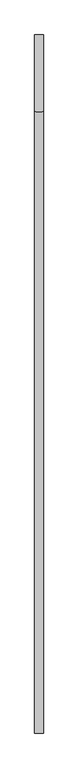
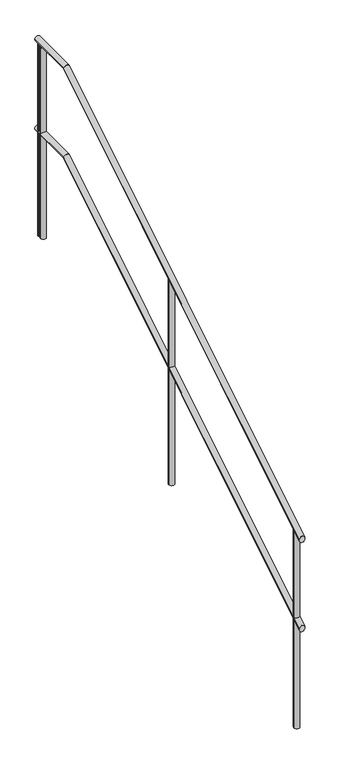
"""IFC4 building model written with IfcOpenShell, lengths in millimetres: railing geometry."""

from ifc_helpers import new_model, si_unit, point, frame, frame_2d, origin, place, context, project, spatial, circle_curve, ellipse_curve, trimmed, segment, composite_curve, outline, extrude, source, transform, mapped, element, save
from ifc_brep_helpers import plane_surface, cylinder_surface, advanced_brep


def railing_c1bf2265(model_context):
    return source(origin(), model_context, "Body", "SolidModel", [
        advanced_brep(
        [(-2206.0, 45684.2482382, -450.9609787), (-2176.0, 45684.2482382, -450.9609787), (-2206.0, 47848.5050237, 885.0), (-2176.0, 47848.5050237, 885.0), (-2206.0, 48114.2482382, 885.0), (-2176.0, 48114.2482382, 885.0)],
        [
            (0, 1, ellipse_curve(frame((-2191.0, 45684.2482382, -450.9609787), z_axis=(0.0, -1.0, 0.0), x_axis=(0.0, 0.0, -1.0)), 17.6276454, 15.0)),
            (1, 0, ellipse_curve(frame((-2191.0, 45684.2482382, -450.9609787), z_axis=(0.0, -1.0, 0.0), x_axis=(0.0, 0.0, -1.0)), 17.6276454, 15.0)),
            (0, 2),
            (2, 3, ellipse_curve(frame((-2191.0, 47848.5050237, 885.0), z_axis=(0.0, -0.9620125025549409, -0.27300539358770887), x_axis=(0.0, 0.27300539358770864, -0.962012502554941)), 15.5923129, 15.0)),
            (3, 1),
            (3, 2, ellipse_curve(frame((-2191.0, 47848.5050237, 885.0), z_axis=(0.0, -0.9620125025549409, -0.27300539358770887), x_axis=(0.0, 0.27300539358770864, -0.962012502554941)), 15.5923129, 15.0)),
            (4, 5, circle_curve(frame((-2191.0, 48114.2482382, 885.0), z_axis=(0.0, 1.0, 0.0), x_axis=(1.0, 0.0, 0.0)), 15.0)),
            (5, 4, circle_curve(frame((-2191.0, 48114.2482382, 885.0), z_axis=(0.0, 1.0, 0.0), x_axis=(1.0, 0.0, 0.0)), 15.0)),
            (2, 4),
            (5, 3),
        ],
        [
            plane_surface(frame((-2191.0, 45684.2482382, -433.3333333), z_axis=(0.0, -1.0, 0.0), x_axis=(0.0, 0.0, 1.0))),
            cylinder_surface(frame((-2191.0, 45692.1272762, -446.097375), z_axis=(0.0, -0.8509361101440404, -0.5252692037926169), x_axis=(1.0, 0.0, 0.0)), 15.0),
            plane_surface(frame((-2191.0, 48114.2482382, 900.0), z_axis=(0.0, 1.0, 0.0), x_axis=(0.0, 0.0, 1.0))),
            cylinder_surface(frame((-2191.0, 47844.2482382, 885.0), z_axis=(0.0, -1.0, 0.0), x_axis=(1.0, 0.0, 0.0)), 15.0),
        ],
        [
            (0, [[1, 2]]),
            (1, [[-1, 3, 4, 5]]),
            (1, [[-2, -5, 6, -3]]),
            (2, [[7, 8]]),
            (3, [[-4, 9, -8, 10]]),
            (3, [[-6, -10, -7, -9]]),
        ],
    ),
        advanced_brep(
        [(-2206.0, 45684.2482382, 49.0390213), (-2176.0, 45684.2482382, 49.0390213), (-2206.0, 47848.5050237, 1385.0), (-2176.0, 47848.5050237, 1385.0), (-2206.0, 48114.2482382, 1385.0), (-2176.0, 48114.2482382, 1385.0)],
        [
            (0, 1, ellipse_curve(frame((-2191.0, 45684.2482382, 49.0390213), z_axis=(0.0, -1.0, 0.0), x_axis=(0.0, 0.0, -1.0)), 17.6276454, 15.0)),
            (1, 0, ellipse_curve(frame((-2191.0, 45684.2482382, 49.0390213), z_axis=(0.0, -1.0, 0.0), x_axis=(0.0, 0.0, -1.0)), 17.6276454, 15.0)),
            (0, 2),
            (2, 3, ellipse_curve(frame((-2191.0, 47848.5050237, 1385.0), z_axis=(0.0, -0.9620125025549409, -0.27300539358770887), x_axis=(0.0, 0.27300539358770864, -0.962012502554941)), 15.5923129, 15.0)),
            (3, 1),
            (3, 2, ellipse_curve(frame((-2191.0, 47848.5050237, 1385.0), z_axis=(0.0, -0.9620125025549409, -0.27300539358770887), x_axis=(0.0, 0.27300539358770864, -0.962012502554941)), 15.5923129, 15.0)),
            (4, 5, circle_curve(frame((-2191.0, 48114.2482382, 1385.0), z_axis=(0.0, 1.0, 0.0), x_axis=(1.0, 0.0, 0.0)), 15.0)),
            (5, 4, circle_curve(frame((-2191.0, 48114.2482382, 1385.0), z_axis=(0.0, 1.0, 0.0), x_axis=(1.0, 0.0, 0.0)), 15.0)),
            (2, 4),
            (5, 3),
        ],
        [
            plane_surface(frame((-2191.0, 45684.2482382, 66.6666667), z_axis=(0.0, -1.0, 0.0), x_axis=(0.0, 0.0, 1.0))),
            cylinder_surface(frame((-2191.0, 45692.1272762, 53.902625), z_axis=(0.0, -0.8509361101440404, -0.5252692037926169), x_axis=(1.0, 0.0, 0.0)), 15.0),
            plane_surface(frame((-2191.0, 48114.2482382, 1400.0), z_axis=(0.0, 1.0, 0.0), x_axis=(0.0, 0.0, 1.0))),
            cylinder_surface(frame((-2191.0, 47844.2482382, 1385.0), z_axis=(0.0, -1.0, 0.0), x_axis=(1.0, 0.0, 0.0)), 15.0),
        ],
        [
            (0, [[1, 2]]),
            (1, [[-1, 3, 4, 5]]),
            (1, [[-2, -5, 6, -3]]),
            (2, [[7, 8]]),
            (3, [[-4, 9, -8, 10]]),
            (3, [[-6, -10, -7, -9]]),
        ],
    ),
        extrude(outline(composite_curve([segment(trimmed(circle_curve(frame_2d((-2191.0, 48084.2482382)), 15.0), [point((-2206.0, 48084.2482382))], [point((-2176.0, 48084.2482382))], False, "CARTESIAN"), True, "CONTINUOUS"), segment(trimmed(circle_curve(frame_2d((-2191.0, 48084.2482382)), 15.0), [point((-2176.0, 48084.2482382))], [point((-2206.0, 48084.2482382))], False, "CARTESIAN"), True, "CONTINUOUS")], self_intersect=False)), frame((0.0, 0.0, 300.0), z_axis=(0.0, 0.0, 1.0), x_axis=(1.0, 0.0, 0.0)), (0.0, 0.0, 1.0), 1070.0),
        advanced_brep(
        [(-2176.0, 46884.2482382, 777.4074074), (-2176.0, 46884.2482382, -366.6666667), (-2206.0, 46884.2482382, -366.6666667), (-2206.0, 46884.2482382, 777.4074074)],
        [
            (0, 1),
            (1, 2, circle_curve(frame((-2191.0, 46884.2482382, -366.6666667), z_axis=(0.0, 0.0, 1.0), x_axis=(-1.0, 0.0, 0.0)), 15.0)),
            (2, 3),
            (3, 0, ellipse_curve(frame((-2191.0, 46884.2482382, 777.4074074), z_axis=(0.0, 0.5252692037926167, -0.8509361101440406), x_axis=(0.0, 0.8509361101440406, 0.5252692037926162)), 17.6276454, 15.0)),
            (0, 3, ellipse_curve(frame((-2191.0, 46884.2482382, 777.4074074), z_axis=(0.0, 0.5252692037926167, -0.8509361101440406), x_axis=(0.0, 0.8509361101440406, 0.5252692037926162)), 17.6276454, 15.0)),
            (2, 1, circle_curve(frame((-2191.0, 46884.2482382, -366.6666667), z_axis=(0.0, 0.0, 1.0), x_axis=(-1.0, 0.0, 0.0)), 15.0)),
        ],
        [
            cylinder_surface(frame((-2191.0, 46884.2482382, -466.6666667), z_axis=(0.0, 0.0, 1.0), x_axis=(-1.0, 0.0, 0.0)), 15.0),
            plane_surface(frame((-2216.0, 46909.2482382, 792.8395062), z_axis=(0.0, -0.5252692037926167, 0.8509361101440406), x_axis=(1.0, 0.0, 0.0))),
            plane_surface(frame((-2216.0, 46859.2482382, -366.6666667), z_axis=(0.0, 0.0, -1.0), x_axis=(1.0, 0.0, 0.0))),
        ],
        [
            (0, [[1, 2, 3, 4]]),
            (0, [[-1, 5, -3, 6]]),
            (1, [[-4, -5]]),
            (2, [[-2, -6]]),
        ],
    ),
        extrude(outline(composite_curve([segment(trimmed(circle_curve(frame_2d((-2191.0, 48064.2482382)), 15.0), [point((-2206.0, 48064.2482382))], [point((-2176.0, 48064.2482382))], False, "CARTESIAN"), True, "CONTINUOUS"), segment(trimmed(circle_curve(frame_2d((-2191.0, 48064.2482382)), 15.0), [point((-2176.0, 48064.2482382))], [point((-2206.0, 48064.2482382))], False, "CARTESIAN"), True, "CONTINUOUS")], self_intersect=False)), frame((0.0, 0.0, 300.0), z_axis=(0.0, 0.0, 1.0), x_axis=(1.0, 0.0, 0.0)), (0.0, 0.0, 1.0), 1070.0),
        advanced_brep(
        [(-2176.0, 45734.2482382, 67.5308642), (-2176.0, 45734.2482382, -1033.3333333), (-2206.0, 45734.2482382, -1033.3333333), (-2206.0, 45734.2482382, 67.5308642)],
        [
            (0, 1),
            (1, 2, circle_curve(frame((-2191.0, 45734.2482382, -1033.3333333), z_axis=(0.0, 0.0, 1.0), x_axis=(-1.0, 0.0, 0.0)), 15.0)),
            (2, 3),
            (3, 0, ellipse_curve(frame((-2191.0, 45734.2482382, 67.5308642), z_axis=(0.0, 0.5252692037926167, -0.8509361101440406), x_axis=(0.0, 0.8509361101440406, 0.5252692037926162)), 17.6276454, 15.0)),
            (0, 3, ellipse_curve(frame((-2191.0, 45734.2482382, 67.5308642), z_axis=(0.0, 0.5252692037926167, -0.8509361101440406), x_axis=(0.0, 0.8509361101440406, 0.5252692037926162)), 17.6276454, 15.0)),
            (2, 1, circle_curve(frame((-2191.0, 45734.2482382, -1033.3333333), z_axis=(0.0, 0.0, 1.0), x_axis=(-1.0, 0.0, 0.0)), 15.0)),
        ],
        [
            cylinder_surface(frame((-2191.0, 45734.2482382, -1133.3333333), z_axis=(0.0, 0.0, 1.0), x_axis=(-1.0, 0.0, 0.0)), 15.0),
            plane_surface(frame((-2216.0, 45759.2482382, 82.962963), z_axis=(0.0, -0.5252692037926167, 0.8509361101440406), x_axis=(1.0, 0.0, 0.0))),
            plane_surface(frame((-2216.0, 45709.2482382, -1033.3333333), z_axis=(0.0, 0.0, -1.0), x_axis=(1.0, 0.0, 0.0))),
        ],
        [
            (0, [[1, 2, 3, 4]]),
            (0, [[-1, 5, -3, 6]]),
            (1, [[-4, -5]]),
            (2, [[-2, -6]]),
        ],
    ),
    ])


if __name__ == "__main__":
    model = new_model("IFC4")
    model_context = context("Model", 3, world=origin())
    ifc_project = project(units=[si_unit("LENGTHUNIT", "METRE", prefix="MILLI")], contexts=[model_context])
    site = spatial("IfcSite", under=ifc_project)
    building = spatial("IfcBuilding", under=site)
    placement = place(None, origin())
    railing_shape = railing_c1bf2265(model_context)
    element("IfcRailing", 1, at=placement, inside=building, context=model_context, shape_type="MappedRepresentation", body=[
        mapped(railing_shape, transform((0.0, 0.0, 0.0), x_axis=(1.0, 0.0, 0.0), y_axis=(0.0, 1.0, 0.0), z_axis=(0.0, 0.0, 1.0))),
    ])
    save(model, "model.ifc")
